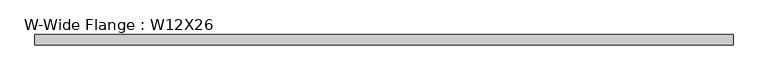
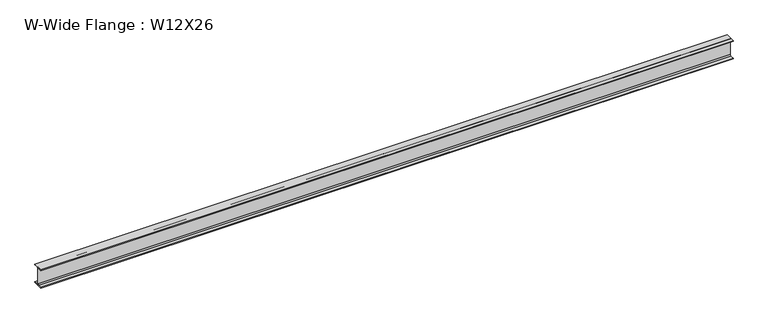
"""IFC4 building model written with IfcOpenShell, lengths in millimetres: beam geometry, W-Wide Flange : W12X26."""

import ifcopenshell
import ifcopenshell.guid

model = None  # the IFC model being written
_history = None  # IfcOwnerHistory: only IFC2X3 demands one
_inside = {}  # id of a spatial element -> (the spatial element, [elements in it])
_under = {}  # id of a project, library or spatial element -> (it, [spatial elements below it])
_declared = {}  # id of a project -> (the project, [libraries it declares])
_typed = {}  # id of a type object -> (the type object, [elements of that type])
_made_of = {}  # id of a material, layer set ... -> (it, [elements and type objects made of it])


def new_model(schema):
    """Start an empty IFC model of exactly this schema.

    Asked for "IFC4X3", IfcOpenShell would pick the latest addendum, in which some entities
    have other attributes; the version numbers below select the first issue.
    IFC2X3 requires an IfcOwnerHistory on every rooted entity: one is made here for all.
    """
    global model, _history
    if schema == "IFC4X3":
        model = ifcopenshell.file(schema_version=(4, 3, 0, 0))
    else:
        model = ifcopenshell.file(schema=schema)
    _inside.clear()
    _under.clear()
    _declared.clear()
    _typed.clear()
    _made_of.clear()
    _history = None
    if model.schema == "IFC2X3":
        org = make("IfcOrganization", Name="unknown")
        user = make(
            "IfcPersonAndOrganization",
            ThePerson=make("IfcPerson", FamilyName="unknown"),
            TheOrganization=org,
        )
        app = make(
            "IfcApplication",
            ApplicationDeveloper=org,
            Version="unknown",
            ApplicationFullName="unknown",
            ApplicationIdentifier="unknown",
        )
        _history = make(
            "IfcOwnerHistory",
            OwningUser=user,
            OwningApplication=app,
            ChangeAction="ADDED",
            CreationDate=0,
        )
    return model


def make(cls, **values):
    """One entity of the class cls with the attributes given. An attribute that is None is left unset."""
    return model.create_entity(
        cls, **{name: value for name, value in values.items() if value is not None}
    )


def rooted(cls, **values):
    """An entity with a GlobalId (a new one), such as an element, a storey or a relation."""
    return make(cls, GlobalId=ifcopenshell.guid.new(), OwnerHistory=_history, **values)


def si_unit(unit_type, name, prefix=None):
    """IfcSIUnit, for example si_unit("LENGTHUNIT", "METRE", prefix="MILLI")."""
    return make("IfcSIUnit", UnitType=unit_type, Prefix=prefix, Name=name)


def assignment(units):
    """IfcUnitAssignment: the units of a project."""
    return None if units is None else make("IfcUnitAssignment", Units=units)


def point(xyz):
    """IfcCartesianPoint."""
    return None if xyz is None else make("IfcCartesianPoint", Coordinates=xyz)


def direction(xyz):
    """IfcDirection."""
    return None if xyz is None else make("IfcDirection", DirectionRatios=xyz)


def frame(location, z_axis=None, x_axis=None):
    """IfcAxis2Placement3D, a coordinate frame: its origin and axes. An axis left out is left unset."""
    return make(
        "IfcAxis2Placement3D",
        Location=point(location),
        Axis=direction(z_axis),
        RefDirection=direction(x_axis),
    )


def frame_2d(location, x_axis=None):
    """IfcAxis2Placement2D, a coordinate frame in the plane: its origin and x axis."""
    return make(
        "IfcAxis2Placement2D", Location=point(location), RefDirection=direction(x_axis)
    )


def origin():
    """The frame at (0, 0, 0) with its axes left unset."""
    return frame((0.0, 0.0, 0.0))


def place(relative_to, where):
    """IfcLocalPlacement: puts the frame where relative to a parent placement (None: the world)."""
    return make(
        "IfcLocalPlacement", PlacementRelTo=relative_to, RelativePlacement=where
    )


def context(
    kind, dimensions, precision=None, world=None, true_north=None, identifier=None
):
    """IfcGeometricRepresentationContext, for example the 3D "Model" context."""
    return make(
        "IfcGeometricRepresentationContext",
        ContextIdentifier=identifier,
        ContextType=kind,
        CoordinateSpaceDimension=dimensions,
        Precision=precision,
        WorldCoordinateSystem=world,
        TrueNorth=true_north,
    )


def project(units=None, contexts=None):
    """IfcProject with its units and contexts."""
    return rooted(
        "IfcProject",
        Name="project",
        RepresentationContexts=contexts,
        UnitsInContext=assignment(units),
    )


def spatial(cls, under=None, at=None, **own):
    """A site, building, storey or space (cls), placed at a placement, below another one or the project."""
    s = rooted(cls, ObjectPlacement=at, **own)
    if under is not None:
        _under.setdefault(under.id(), (under, []))[1].append(s)
    return s


def polyline(points):
    """IfcPolyline through the points."""
    return make("IfcPolyline", Points=[point(p) for p in points])


def circle_curve(where, radius):
    """IfcCircle in the frame where."""
    return make("IfcCircle", Position=where, Radius=radius)


def trimmed(basis, trim1, trim2, sense, master):
    """IfcTrimmedCurve: the piece of a basis curve between two trims."""
    return make(
        "IfcTrimmedCurve",
        BasisCurve=basis,
        Trim1=trim1,
        Trim2=trim2,
        SenseAgreement=sense,
        MasterRepresentation=master,
    )


def segment(curve, same_sense, transition):
    """IfcCompositeCurveSegment."""
    return make(
        "IfcCompositeCurveSegment",
        Transition=transition,
        SameSense=same_sense,
        ParentCurve=curve,
    )


def composite_curve(segments, self_intersect=None):
    """IfcCompositeCurve: segments joined end to end."""
    return make("IfcCompositeCurve", Segments=segments, SelfIntersect=self_intersect)


def outline(outer, holes=None, kind="AREA"):
    """IfcArbitraryClosedProfileDef: a profile drawn as a closed curve; with holes, ...WithVoids."""
    if holes is None:
        return make("IfcArbitraryClosedProfileDef", ProfileType=kind, OuterCurve=outer)
    return make(
        "IfcArbitraryProfileDefWithVoids",
        ProfileType=kind,
        OuterCurve=outer,
        InnerCurves=holes,
    )


def extrude(swept, where, along, depth):
    """IfcExtrudedAreaSolid: the profile swept, set in the frame where, extruded along a direction by depth."""
    return make(
        "IfcExtrudedAreaSolid",
        SweptArea=swept,
        Position=where,
        ExtrudedDirection=direction(along),
        Depth=depth,
    )


def shape(context_of_items, identifier, shape_type, items):
    """IfcShapeRepresentation: the items that make up one representation, for example the "Body"."""
    return make(
        "IfcShapeRepresentation",
        ContextOfItems=context_of_items,
        RepresentationIdentifier=identifier,
        RepresentationType=shape_type,
        Items=items,
    )


def source(mapping_origin, context_of_items, identifier, shape_type, items):
    """IfcRepresentationMap: a shape defined once, which mapped items show again and again."""
    return make(
        "IfcRepresentationMap",
        MappingOrigin=mapping_origin,
        MappedRepresentation=shape(context_of_items, identifier, shape_type, items),
    )


def transform(
    local_origin,
    x_axis=None,
    y_axis=None,
    z_axis=None,
    scale=None,
    scale2=None,
    scale3=None,
    uniform=True,
):
    """IfcCartesianTransformationOperator3D, or its non-uniform kind. x_axis, y_axis, z_axis: its Axis1, 2, 3."""
    if uniform:
        return make(
            "IfcCartesianTransformationOperator3D",
            Axis1=direction(x_axis),
            Axis2=direction(y_axis),
            LocalOrigin=point(local_origin),
            Scale=scale,
            Axis3=direction(z_axis),
        )
    return make(
        "IfcCartesianTransformationOperator3DnonUniform",
        Axis1=direction(x_axis),
        Axis2=direction(y_axis),
        LocalOrigin=point(local_origin),
        Scale=scale,
        Axis3=direction(z_axis),
        Scale2=scale2,
        Scale3=scale3,
    )


def mapped(mapping_source, mapping_target):
    """IfcMappedItem: shows the shape of a source again, moved by a transform."""
    return make(
        "IfcMappedItem", MappingSource=mapping_source, MappingTarget=mapping_target
    )


def made_of(thing, what):
    """Note that an element or type object is made of a material, layer set ...; save() writes the relation."""
    if what is not None:
        _made_of.setdefault(what.id(), (what, []))[1].append(thing)
    return thing


def element(
    cls,
    number,
    at=None,
    inside=None,
    cuts=None,
    type_object=None,
    material=None,
    context=None,
    identifier="Body",
    shape_type=None,
    held_by="IfcProductDefinitionShape",
    body=None,
    shapes=None,
    **own,
):
    """One element of the class cls, such as IfcWall. Its Tag is "e" and its number.

    at: its placement. inside: the storey or other place that contains it. cuts: it is an
    opening in that element (IfcRelVoidsElement). A single representation is given by context,
    identifier, shape_type and body (its items); several are given by shapes. held_by: the class
    of the entity that holds the representations. save() writes the other relations.
    """
    e = rooted(cls, Tag="e%d" % number, ObjectPlacement=at, **own)
    if body is not None:
        shapes = [shape(context, identifier, shape_type, body)]
    if shapes is not None:
        e.Representation = make(held_by, Representations=shapes)
    if inside is not None:
        _inside.setdefault(inside.id(), (inside, []))[1].append(e)
    if cuts is not None:
        rooted(
            "IfcRelVoidsElement", RelatingBuildingElement=cuts, RelatedOpeningElement=e
        )
    if type_object is not None:
        _typed.setdefault(type_object.id(), (type_object, []))[1].append(e)
    return made_of(e, material)


def aggregate(whole, parts):
    """IfcRelAggregates: a whole, such as a stair, and the parts it consists of."""
    return rooted("IfcRelAggregates", RelatingObject=whole, RelatedObjects=parts)


def save(model, path):
    """Write the relations noted so far, then the file.

    IfcRelAggregates (storeys below a building ...), IfcRelContainedInSpatialStructure (elements
    in a storey), IfcRelDefinesByType, IfcRelAssociatesMaterial and IfcRelDeclares: one each for
    every whole, place, type object, material and project.
    """
    for whole, parts in _under.values():
        aggregate(whole, parts)
    for where, things in _inside.values():
        rooted(
            "IfcRelContainedInSpatialStructure",
            RelatedElements=things,
            RelatingStructure=where,
        )
    for kind, things in _typed.values():
        rooted("IfcRelDefinesByType", RelatedObjects=things, RelatingType=kind)
    for what, things in _made_of.values():
        rooted("IfcRelAssociatesMaterial", RelatedObjects=things, RelatingMaterial=what)
    for by, libraries in _declared.values():
        rooted("IfcRelDeclares", RelatingContext=by, RelatedDefinitions=libraries)
    model.write(path)


def w_wide_flange_w12x26_16ae085f(model_context):
    return source(origin(), model_context, "Body", "SweptSolid", [
        extrude(outline(composite_curve([segment(polyline([(82.4011719, -145.5539063), (82.4011719, -155.178125), (-82.4011719, -155.178125), (-82.4011719, -145.5539063), (-20.2902344, -145.5539063)]), True, "CONTINUOUS"), segment(trimmed(circle_curve(frame_2d((-20.2902344, -128.190625)), 17.3632812), [point((-20.2902344, -145.5539063))], [point((-2.9269531, -128.190625))], True, "CARTESIAN"), True, "CONTINUOUS"), segment(polyline([(-2.9269531, -128.190625), (-2.9269531, 128.190625)]), True, "CONTINUOUS"), segment(trimmed(circle_curve(frame_2d((-20.2902344, 128.190625)), 17.3632812), [point((-2.9269531, 128.190625))], [point((-20.2902344, 145.5539062))], True, "CARTESIAN"), True, "CONTINUOUS"), segment(polyline([(-20.2902344, 145.5539062), (-82.4011719, 145.5539062), (-82.4011719, 155.178125), (82.4011719, 155.178125), (82.4011719, 145.5539062), (20.2902344, 145.5539062)]), True, "CONTINUOUS"), segment(trimmed(circle_curve(frame_2d((20.2902344, 128.190625)), 17.3632812), [point((20.2902344, 145.5539062))], [point((2.9269531, 128.190625))], True, "CARTESIAN"), True, "CONTINUOUS"), segment(polyline([(2.9269531, 128.190625), (2.9269531, -128.190625)]), True, "CONTINUOUS"), segment(trimmed(circle_curve(frame_2d((20.2902344, -128.190625)), 17.3632812), [point((2.9269531, -128.190625))], [point((20.2902344, -145.5539063))], True, "CARTESIAN"), True, "CONTINUOUS"), segment(polyline([(20.2902344, -145.5539063), (82.4011719, -145.5539063)]), True, "CONTINUOUS")], self_intersect=False)), frame((-5629.6972349, 0.0, 0.0), z_axis=(1.0, 0.0, 0.0), x_axis=(0.0, 1.0, 0.0)), (0.0, 0.0, 1.0), 11259.3944699),
    ])


if __name__ == "__main__":
    model = new_model("IFC4")
    model_context = context("Model", 3, world=origin())
    ifc_project = project(units=[si_unit("LENGTHUNIT", "METRE", prefix="MILLI")], contexts=[model_context])
    site = spatial("IfcSite", under=ifc_project)
    building = spatial("IfcBuilding", under=site)
    placement = place(None, origin())
    w_wide_flange_w12x26_shape = w_wide_flange_w12x26_16ae085f(model_context)
    element("IfcBeam", 1, ObjectType="W-Wide Flange : W12X26", at=placement, inside=building, context=model_context, shape_type="MappedRepresentation", body=[
        mapped(w_wide_flange_w12x26_shape, transform((0.0, 0.0, 0.0), x_axis=(1.0, 0.0, 0.0), y_axis=(0.0, 1.0, 0.0), z_axis=(0.0, 0.0, 1.0))),
    ])
    save(model, "model.ifc")

# Revit data of these elements
# Type "W-Wide Flange : W12X26"
#   Assembly Code = "B10"
#   W = 26
#   Length [instance default] = 5' - 0"
#   bf = 0' - 6 125/256"
#   d = 1' - 0 7/32"
#   k = 0' - 1 1/16"
#   k2 = 0' - 0 175/256"
#   tf = 0' - 0 97/256"
#   tw = 0' - 0 59/256"
#   A = 0.053125 SF
#   Structural Material [instance default] = none
# Element 1 (IfcBeam, "W-Wide Flange : W12X26")
#   Structural Material = Dark metal
#   Materials on its faces: "Dark metal"
# Materials
#   "Dark metal": class "Generic", colour RGB 44 29 29, transparency 0, Cost = 0
